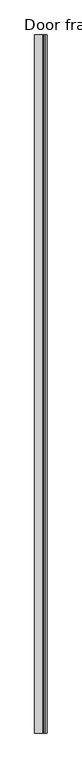
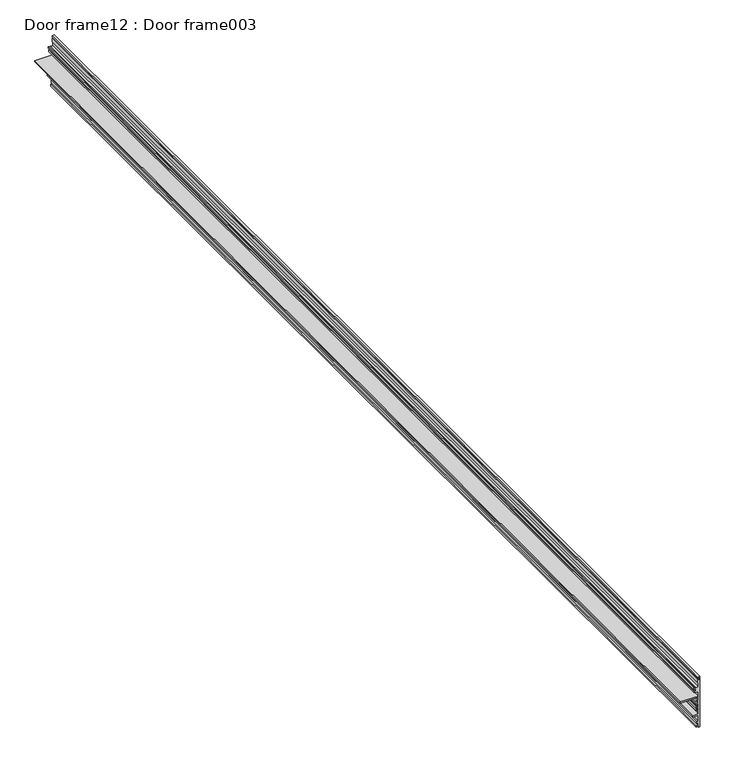
"""IFC4 building model written with IfcOpenShell, lengths in millimetres: proxy geometry, Door frame12 : Door frame003."""

from ifc_helpers import new_model, si_unit, frame, origin, place, context, project, spatial, polyline, outline, extrude, source, transform, mapped, element, save


def door_frame12_door_frame003_8b51607b(model_context):
    return source(origin(), model_context, "Body", "SweptSolid", [
        extrude(outline(polyline([(36640.7292623, 15558.7942271), (36638.6348329, 15558.7942271), (36638.6348329, 15555.2376968), (36635.0786991, 15555.2376968), (36635.0786991, 15556.6349454), (36637.237374, 15556.6349454), (36637.237374, 15558.7933141), (36629.3636227, 15558.7933141), (36629.3636227, 15556.634085), (36631.522833, 15556.634085), (36631.522833, 15555.2366262), (36627.9663742, 15555.2366262), (36627.9663742, 15558.7925325), (36625.8711226, 15558.7925325), (36625.8711226, 15556.6360862), (36624.9183358, 15554.7312296), (36623.9664094, 15556.636373), (36623.9664094, 15558.7925159), (36617.0240434, 15558.7925159), (36617.0240434, 15549.0103859), (36613.8490434, 15549.0103859), (36613.8490434, 15558.7893859), (36602.905231, 15558.7893859), (36602.905231, 15556.3015659), (36598.5961003, 15556.3015659), (36600.1211436, 15558.8008339), (36594.775583, 15558.8008339), (36595.6486981, 15555.544285), (36592.4137824, 15555.2607758), (36593.5561506, 15557.6006351), (36593.5561506, 15558.9588558), (36591.6240434, 15558.9588558), (36591.6240434, 15561.9764133), (36686.8713846, 15561.9764133), (36686.8713846, 15557.8513976), (36684.2230088, 15557.8513976), (36684.2230088, 15559.1060732), (36685.5545864, 15559.1060732), (36685.5545864, 15560.591093), (36680.6298938, 15560.591093), (36680.6298938, 15559.1060732), (36681.9249044, 15559.1060732), (36681.9249044, 15557.8513976), (36675.7714394, 15557.8513976), (36675.7714394, 15559.0526143), (36667.7720071, 15559.0526143), (36667.7720071, 15554.3561718), (36667.5392258, 15553.1571189), (36668.6824408, 15550.8176037), (36665.4474399, 15551.1001389), (36666.3193526, 15554.3561219), (36660.9960694, 15554.3561219), (36662.4395074, 15551.856014), (36658.8017047, 15551.856014), (36658.8017047, 15558.7960921), (36650.6101085, 15558.7960921), (36650.6101085, 15527.0514077), (36648.0323358, 15527.0514077), (36648.0323358, 15558.795388), (36642.634549, 15558.795388), (36642.634549, 15556.636373), (36641.6823358, 15554.7312296), (36640.7292623, 15556.6360862), (36640.7292623, 15558.7942271)])), frame((0.0, -1052.8906567, 0.0), z_axis=(0.0, 1.0, 0.0), x_axis=(0.0, 0.0, 1.0)), (0.0, 0.0, 1.0), 1999.85),
    ])


if __name__ == "__main__":
    model = new_model("IFC4")
    model_context = context("Model", 3, world=origin())
    ifc_project = project(units=[si_unit("LENGTHUNIT", "METRE", prefix="MILLI")], contexts=[model_context])
    site = spatial("IfcSite", under=ifc_project)
    building = spatial("IfcBuilding", under=site)
    placement = place(None, origin())
    door_frame12_door_frame003_shape = door_frame12_door_frame003_8b51607b(model_context)
    element("IfcBuildingElementProxy", 1, Name="Door frame12 : Door frame003", ObjectType="Door frame12 : Door frame003", at=placement, inside=building, context=model_context, shape_type="MappedRepresentation", body=[
        mapped(door_frame12_door_frame003_shape, transform((0.0, 0.0, 0.0), x_axis=(1.0, 0.0, 0.0), y_axis=(0.0, 1.0, 0.0), z_axis=(0.0, 0.0, 1.0))),
    ])
    save(model, "model.ifc")

# Revit data of these elements
# Type "Door frame12 : Door frame003"
#   NameOverride = "Door frame003"
# Element 1 (IfcBuildingElementProxy, "Door frame12 : Door frame003")
#   Materials on its faces: "FLEETWOOD SERIES T-3200 SINGLE SWING DOOR FRAME"
# Materials
#   "FLEETWOOD SERIES T-3200 SINGLE SWING DOOR FRAME": class "Unassigned", colour RGB 128 128 128, transparency 0, Cost = 0
